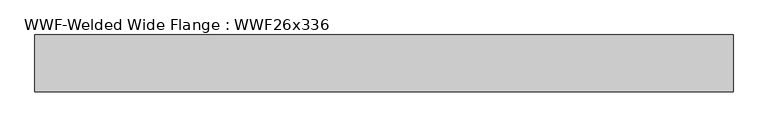
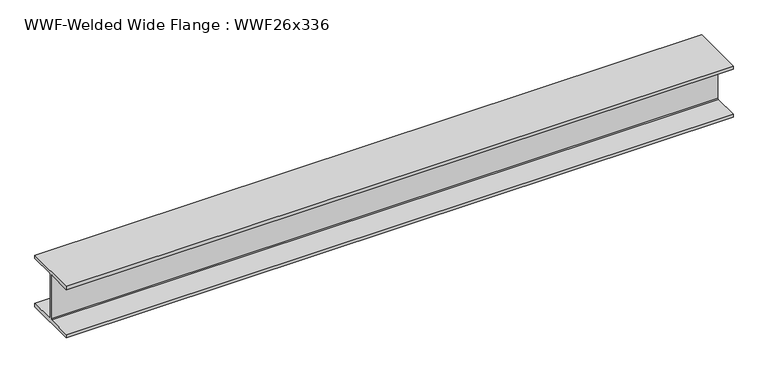
"""IFC4 building model written with IfcOpenShell, lengths in millimetres: beam geometry, WWF-Welded Wide Flange : WWF26x336."""

from ifc_helpers import new_model, si_unit, frame, origin, place, context, project, spatial, polyline, outline, extrude, source, transform, mapped, element, save


def wwf_welded_wide_flange_wwf26x336_65f30c1f(model_context):
    return source(origin(), model_context, "Body", "SweptSolid", [
        extrude(outline(polyline([(324.993, -284.988), (324.993, -324.993), (-324.993, -324.993), (-324.993, -284.988), (-20.6375, -284.988), (-9.9949, -274.3454), (-9.9949, 274.3454), (-20.6375, 284.988), (-324.993, 284.988), (-324.993, 324.993), (324.993, 324.993), (324.993, 284.988), (20.6375, 284.988), (9.9949, 274.3454), (9.9949, -274.3454), (20.6375, -284.988), (324.993, -284.988)])), frame((-3827.7582557, 0.0, 0.0), z_axis=(1.0, 0.0, 0.0), x_axis=(0.0, 1.0, 0.0)), (0.0, 0.0, 1.0), 7985.2438859),
    ])


if __name__ == "__main__":
    model = new_model("IFC4")
    model_context = context("Model", 3, world=origin())
    ifc_project = project(units=[si_unit("LENGTHUNIT", "METRE", prefix="MILLI")], contexts=[model_context])
    site = spatial("IfcSite", under=ifc_project)
    building = spatial("IfcBuilding", under=site)
    placement = place(None, origin())
    wwf_welded_wide_flange_wwf26x336_shape = wwf_welded_wide_flange_wwf26x336_65f30c1f(model_context)
    element("IfcBeam", 1, ObjectType="WWF-Welded Wide Flange : WWF26x336", at=placement, inside=building, context=model_context, shape_type="MappedRepresentation", body=[
        mapped(wwf_welded_wide_flange_wwf26x336_shape, transform((0.0, 0.0, 0.0), x_axis=(1.0, 0.0, 0.0), y_axis=(0.0, 1.0, 0.0), z_axis=(0.0, 0.0, 1.0))),
    ])
    save(model, "model.ifc")

# Revit data of these elements
# Type "WWF-Welded Wide Flange : WWF26x336"
#   Assembly Code = "B10"
#   Nominal d = "12"
#   W = 336
#   Length [instance default] = 1524 mm
#   bf = 649.986 mm
#   d = 649.986 mm
#   k = 20.638 mm
#   tf = 40.005 mm
#   tw = 19.99 mm
#   A = 0.0635483 m²
#   Structural Material [instance default] = Steel ASTM A572
# Element 1 (IfcBeam, "WWF-Welded Wide Flange : WWF26x336")
#   Structural Material = Metal - Steel 43-275
#   Materials on its faces: "Metal - Steel 43-275"
# Materials
#   "Steel ASTM A572": class "Metal", colour RGB 247 247 247, transparency 0, Description = "Structural steel, high strength low alloy, ASTM - A572 - 50", Cost = 0
#   "Metal - Steel 43-275": class "Metal", colour RGB 247 247 247, transparency 0, Cost = 0
